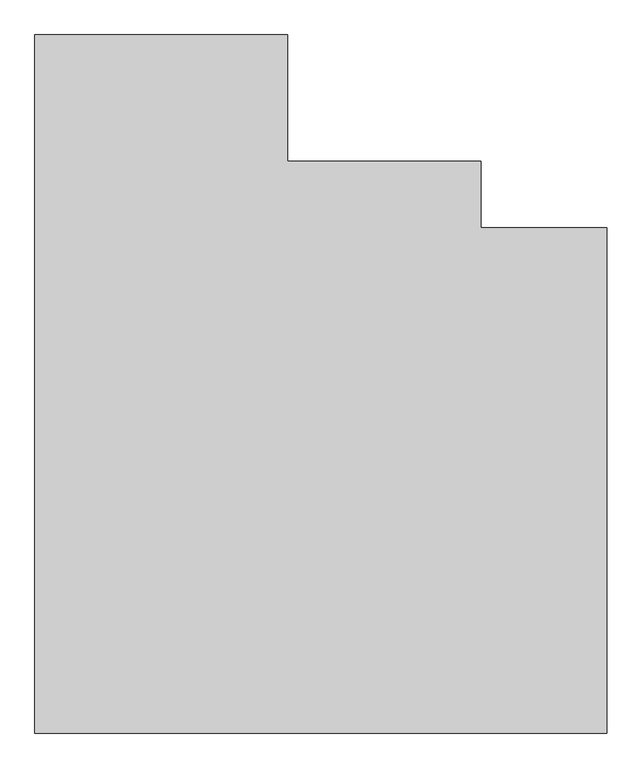
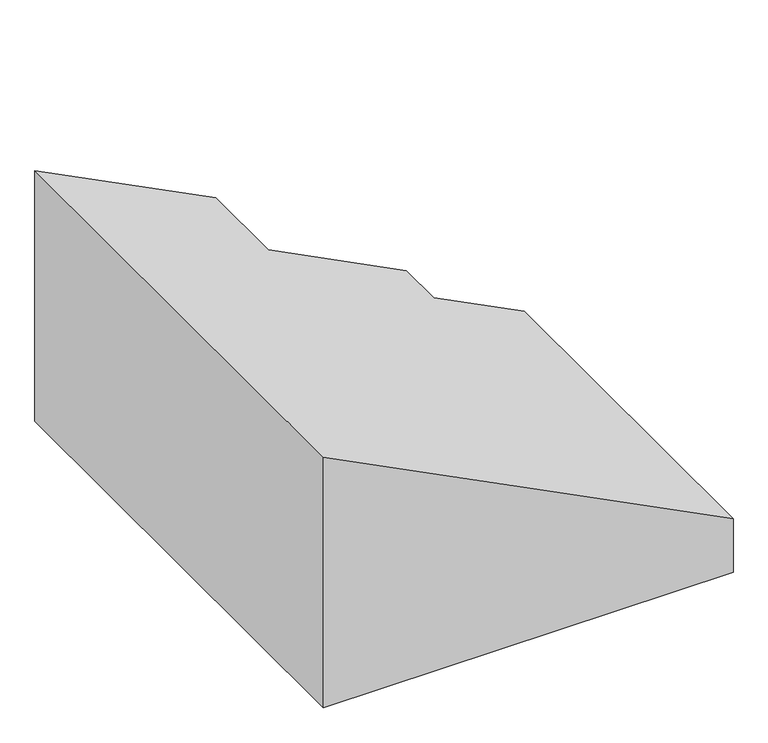
"""IFC4 building model written with IfcOpenShell, lengths in millimetres: proxy geometry, 0_3d."""

from ifc_helpers import new_model, si_unit, origin, place, context, project, spatial, faceted_brep, source, transform, mapped, element, save


def generic_models_dd3d14e7(model_context):
    return source(origin(), model_context, "Body", "Brep", [
        faceted_brep([(4650.0, 0.0, 638.6196708), (4650.0, 4105.0, 638.6196708), (3625.0, 4105.0, 1160.8832565), (3625.0, 4645.0, 1160.8832565), (2055.0, 4645.0, 1960.8382122), (2055.0, 5670.0, 1960.8382122), (0.0, 5670.0, 3007.913011), (0.0, 0.0, 3007.913011), (2055.0, 4645.0, 0.0), (2055.0, 5670.0, 0.0), (3625.0, 4645.0, 0.0), (3625.0, 4105.0, 0.0), (4650.0, 4105.0, 0.0), (4650.0, 0.0, 0.0), (0.0, 0.0, 0.0), (0.0, 5670.0, 0.0)], [[[0, 1, 2, 3, 4, 5, 6, 7]], [[5, 4, 8, 9]], [[4, 3, 10, 8]], [[3, 2, 11, 10]], [[2, 1, 12, 11]], [[1, 0, 13, 12]], [[0, 7, 14, 13]], [[15, 14, 7, 6]], [[6, 5, 9, 15]], [[11, 12, 13, 14, 15, 9, 8, 10]]]),
    ])


if __name__ == "__main__":
    model = new_model("IFC4")
    model_context = context("Model", 3, world=origin())
    ifc_project = project(units=[si_unit("LENGTHUNIT", "METRE", prefix="MILLI")], contexts=[model_context])
    site = spatial("IfcSite", under=ifc_project)
    building = spatial("IfcBuilding", under=site)
    placement = place(None, origin())
    generic_models_shape = generic_models_dd3d14e7(model_context)
    element("IfcBuildingElementProxy", 1, Name="0_3d", ObjectType="0_3d", at=placement, inside=building, context=model_context, shape_type="MappedRepresentation", body=[
        mapped(generic_models_shape, transform((0.0, 0.0, 0.0), x_axis=(1.0, 0.0, 0.0), y_axis=(0.0, 1.0, 0.0), z_axis=(0.0, 0.0, 1.0))),
    ])
    save(model, "model.ifc")

# Revit data of these elements
# Element 1 (IfcBuildingElementProxy, "0_3d")
#   Materials on its faces: "*1"
# Materials
#   "*1": class "Unassigned", colour RGB 175 175 175, transparency 0
